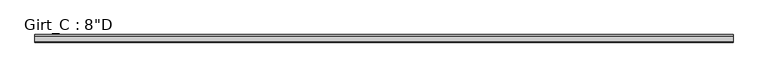
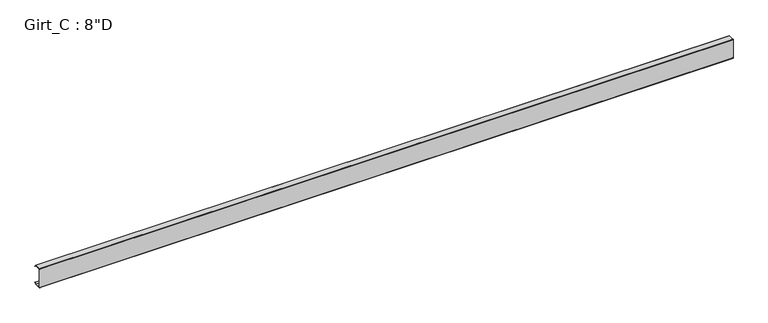
"""IFC4 building model written with IfcOpenShell, lengths in millimetres: beam geometry."""

from ifc_helpers import new_model, si_unit, point, frame, frame_2d, origin, place, context, project, spatial, polyline, circle_curve, trimmed, segment, composite_curve, outline, extrude, source, transform, mapped, element, save


def beam_c55e893e(model_context):
    return source(origin(), model_context, "Body", "SweptSolid", [
        extrude(outline(composite_curve([segment(polyline([(63.5, 101.6), (75.745104, 87.0068534), (73.6169367, 85.221109), (62.204539, 98.821875), (3.3005807, 98.821875)]), True, "CONTINUOUS"), segment(trimmed(circle_curve(frame_2d((3.3741066, 96.8381931)), 1.9850441), [point((3.3005807, 98.821875))], [point((1.3890625, 96.8381931))], True, "CARTESIAN"), True, "CONTINUOUS"), segment(polyline([(1.3890625, 96.8381931), (1.3890625, -96.8389339)]), True, "CONTINUOUS"), segment(trimmed(circle_curve(frame_2d((3.3748024, -96.8389339)), 1.9857399), [point((1.3890625, -96.8389339))], [point((3.2694106, -98.821875))], True, "CARTESIAN"), True, "CONTINUOUS"), segment(polyline([(3.2694106, -98.821875), (62.204539, -98.821875), (73.6169367, -85.221109), (75.745104, -87.0068534), (63.5, -101.6), (3.3734375, -101.6)]), True, "CONTINUOUS"), segment(trimmed(circle_curve(frame_2d((3.3734375, -96.8375)), 4.7625), [point((3.3734375, -101.6))], [point((-1.3890625, -96.8375))], False, "CARTESIAN"), True, "CONTINUOUS"), segment(polyline([(-1.3890625, -96.8375), (-1.3890625, 96.8375)]), True, "CONTINUOUS"), segment(trimmed(circle_curve(frame_2d((3.3734375, 96.8375)), 4.7625), [point((-1.3890625, 96.8375))], [point((3.3734375, 101.6))], False, "CARTESIAN"), True, "CONTINUOUS"), segment(polyline([(3.3734375, 101.6), (63.5, 101.6)]), True, "CONTINUOUS")], self_intersect=False)), frame((-3632.2, 0.0, 0.0), z_axis=(1.0, 0.0, 0.0), x_axis=(0.0, 1.0, 0.0)), (0.0, 0.0, 1.0), 7023.1),
    ])


if __name__ == "__main__":
    model = new_model("IFC4")
    model_context = context("Model", 3, world=origin())
    ifc_project = project(units=[si_unit("LENGTHUNIT", "METRE", prefix="MILLI")], contexts=[model_context])
    site = spatial("IfcSite", under=ifc_project)
    building = spatial("IfcBuilding", under=site)
    placement = place(None, origin())
    beam_shape = beam_c55e893e(model_context)
    element("IfcBeam", 1, ObjectType="Girt_C : 8\"D", at=placement, inside=building, context=model_context, shape_type="MappedRepresentation", body=[
        mapped(beam_shape, transform((0.0, 0.0, 0.0), x_axis=(1.0, 0.0, 0.0), y_axis=(0.0, 1.0, 0.0), z_axis=(0.0, 0.0, 1.0))),
    ])
    save(model, "model.ifc")

# Revit data of these elements
# Type "Girt_C : 8\"D"
#   Web_Thickness = 0' - 0 7/64"
#   Length [instance default] = 10' - 0"
#   Leg_1 = 0' - 2 1/2"
#   Height = 0' - 8"
#   Structural Material [instance default] = none
# Element 1 (IfcBeam, "Girt_C : 8\"D")
#   Structural Material = Steel
#   Materials on its faces: "Steel"
# Materials
#   "Steel": class "Metal", colour RGB 118 118 114, transparency 0, Description = "Steel, mill finish", Cost = 0
